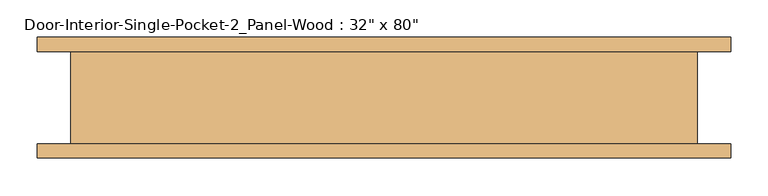
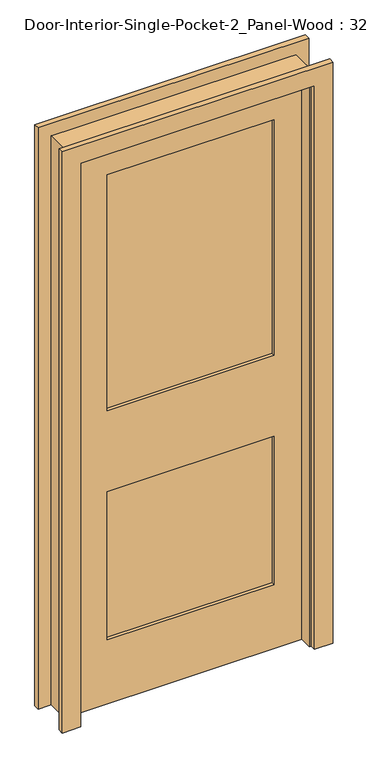
"""IFC4 building model written with IfcOpenShell, lengths in millimetres: door geometry."""

from ifc_helpers import new_model, si_unit, frame, origin, place, context, project, spatial, polyline, outline, extrude, faceted_brep, source, transform, mapped, element, save


def door_810b4294(model_context):
    return source(origin(), model_context, "Body", "SolidModel", [
        extrude(outline(polyline([(0.0, 387.35), (0.0, 450.85), (2101.85, 450.85), (2101.85, -476.25), (0.0, -476.25), (0.0, -412.75), (2038.35, -412.75), (2038.35, 387.35), (0.0, 387.35)])), frame((0.0, -80.9625, 0.0), z_axis=(0.0, 1.0, 0.0), x_axis=(0.0, 0.0, 1.0)), (0.0, 0.0, 1.0), 19.05),
        extrude(outline(polyline([(0.0, 387.35), (0.0, 450.85), (2101.85, 450.85), (2101.85, -476.25), (0.0, -476.25), (0.0, -412.75), (2038.35, -412.75), (2038.35, 387.35), (0.0, 387.35)])), frame((0.0, 61.9125, 0.0), z_axis=(0.0, 1.0, 0.0), x_axis=(0.0, 0.0, 1.0)), (0.0, 0.0, 1.0), 19.05),
        faceted_brep([(406.4, -61.9125, 0.0), (406.4, -17.4625, 0.0), (406.4, -17.4625, 2032.0), (406.4, 17.4625, 2032.0), (406.4, 17.4625, 0.0), (406.4, 61.9125, 0.0), (406.4, 61.9125, 2057.4), (406.4, -61.9125, 2057.4), (-431.8, -61.9125, 2057.4), (-431.8, -61.9125, 0.0), (-406.4, -61.9125, 0.0), (-406.4, -61.9125, 2032.0), (381.0, -61.9125, 2032.0), (381.0, -61.9125, 0.0), (-406.4, 61.9125, 2032.0), (381.0, 61.9125, 2032.0), (381.0, 17.4625, 2032.0), (381.0, -17.4625, 2032.0), (381.0, 61.9125, 0.0), (-406.4, 61.9125, 0.0), (-431.8, 61.9125, 0.0), (-431.8, 61.9125, 2057.4), (381.0, -17.4625, 0.0), (381.0, 17.4625, 0.0)], [[[0, 1, 2, 3, 4, 5, 6, 7]], [[0, 7, 8, 9, 10, 11, 12, 13]], [[11, 14, 15, 16, 3, 2, 17, 12]], [[6, 5, 18, 15, 14, 19, 20, 21]], [[6, 21, 8, 7]], [[10, 9, 20, 19]], [[11, 10, 19, 14]], [[9, 8, 21, 20]], [[1, 0, 13, 22]], [[5, 4, 23, 18]], [[18, 23, 16, 15]], [[23, 4, 3, 16]], [[1, 22, 17, 2]], [[22, 13, 12, 17]]]),
        extrude(outline(polyline([(285.75, -5.8208333), (-285.75, -5.8208333), (-285.75, 5.8208333), (285.75, 5.8208333), (285.75, -5.8208333)])), frame((0.0, 0.0, 1060.45), z_axis=(0.0, 0.0, 1.0), x_axis=(1.0, 0.0, 0.0)), (0.0, 0.0, 1.0), 852.4875),
        extrude(outline(polyline([(285.75, -5.8208333), (-285.75, -5.8208333), (-285.75, 5.8208333), (285.75, 5.8208333), (285.75, -5.8208333)])), frame((0.0, 0.0, 231.775), z_axis=(0.0, 0.0, 1.0), x_axis=(1.0, 0.0, 0.0)), (0.0, 0.0, 1.0), 536.575),
        extrude(outline(polyline([(2032.0, -406.4), (0.0, -406.4), (0.0, 406.4), (2032.0, 406.4), (2032.0, -406.4)]), holes=[polyline([(1912.9375, -285.75), (1912.9375, 285.75), (1060.45, 285.75), (1060.45, -285.75), (1912.9375, -285.75)]), polyline([(768.35, -285.75), (768.35, 285.75), (231.775, 285.75), (231.775, -285.75), (768.35, -285.75)])]), frame((0.0, -17.4625, 0.0), z_axis=(0.0, 1.0, 0.0), x_axis=(0.0, 0.0, 1.0)), (0.0, 0.0, 1.0), 34.925),
    ])


if __name__ == "__main__":
    model = new_model("IFC4")
    model_context = context("Model", 3, world=origin())
    ifc_project = project(units=[si_unit("LENGTHUNIT", "METRE", prefix="MILLI")], contexts=[model_context])
    site = spatial("IfcSite", under=ifc_project)
    building = spatial("IfcBuilding", under=site)
    placement = place(None, origin())
    door_shape = door_810b4294(model_context)
    element("IfcDoor", 1, ObjectType="Door-Interior-Single-Pocket-2_Panel-Wood : 32\" x 80\"", at=placement, inside=building, context=model_context, shape_type="MappedRepresentation", body=[
        mapped(door_shape, transform((0.0, 0.0, 0.0), x_axis=(1.0, 0.0, 0.0), y_axis=(0.0, 1.0, 0.0), z_axis=(0.0, 0.0, 1.0))),
    ])
    save(model, "model.ifc")

# Revit data of these elements
# Type "Door-Interior-Single-Pocket-2_Panel-Wood : 32\" x 80\""
#   Type Mark = "91"
#   COBie.Type.CreatedBy = "doug.wood@us.ibm.com"
#   COBie.Type.CreatedOn = "2016-04-14T02:07:24"
#   COBie.Type.Name = "Doors_Door-Interior-Single-Pocket-2_Panel-Wood_32\" x 80\"_91"
#   COBie.Type.Category = "23-30 10 00 : Doors"
#   COBie.Type.Description = "Door-Interior-Single-Pocket-2_Panel-Wood_32\" x 80\""
#   COBie.Type.Manufacturer = ""
#   COBie.Type.ModelNumber = ""
#   Assembly Code = "C1020300"
#   Analytic Construction = "Wooden"
#   COBie.Type.ReplacementCost = 0
#   Top Rail = 0' - 4 11/16"
#   Thickness = 0' - 1 3/8"
#   Thermal Resistance (R) = 0.455703 (m²·K)/W
#   Stiles = 0' - 4 3/4"
#   Rough Width = 5' - 5"
#   Rough Height = 7' - 0 1/2"
#   Lock Rail = 0' - 7 1/2"
#   Location [instance default] = 2' - 8"
#   Height = 6' - 8"
#   Width = 2' - 8"
#   Heat Transfer Coefficient (U) = 2.19465 W/(m²·K)
#   Bottom Rail = 0' - 9 1/8"
#   COBie.Type = no
#   Panel Open [instance default] = no
#   Trim Material = Trim - White
#   Panel Material = Door - Panel - White
#   Frame Material = Door - Frame - White
#   Visual Light Transmittance = 0
#   Solar Heat Gain Coefficient = 0
#   Wall Closure = (empty or 0)
#   Function = (empty or 0)
# Element 1 (IfcDoor, "Door-Interior-Single-Pocket-2_Panel-Wood : 32\" x 80\"")
#   Materials on its faces: "Door - Panel - White", "Trim - White", "Door - Frame - White"
# Materials
#   "Trim - White": class "Wood", colour RGB 255 255 255, transparency 0, Cost = 0
#   "Door - Panel - White": class "Wood", colour RGB 255 255 255, transparency 0, Cost = 0
#   "Door - Frame - White": class "Miscellaneous", colour RGB 255 255 255, transparency 0, Cost = 0
